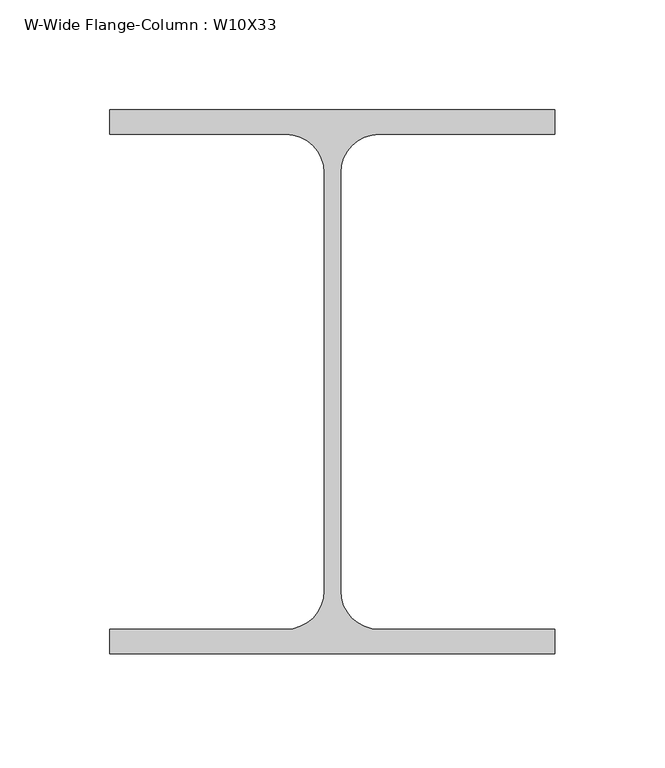
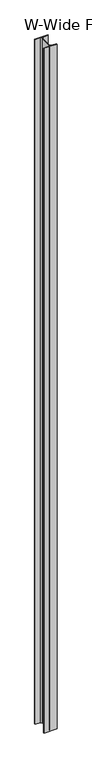
"""IFC4 building model written with IfcOpenShell, lengths in millimetres: column geometry, W-Wide Flange-Column : W10X33."""

from ifc_helpers import new_model, si_unit, point, frame, frame_2d, origin, place, context, project, spatial, polyline, circle_curve, trimmed, segment, composite_curve, outline, extrude, source, transform, mapped, element, save


def w_wide_flange_column_w10x33_06541e1f(model_context):
    return source(origin(), model_context, "Body", "SweptSolid", [
        extrude(outline(composite_curve([segment(polyline([(101.092, -123.571), (-101.092, -123.571), (-101.092, -112.522), (-21.209, -112.522)]), True, "CONTINUOUS"), segment(trimmed(circle_curve(frame_2d((-21.209, -94.996)), 17.526), [point((-21.209, -112.522))], [point((-3.683, -94.996))], True, "CARTESIAN"), True, "CONTINUOUS"), segment(polyline([(-3.683, -94.996), (-3.683, 94.996)]), True, "CONTINUOUS"), segment(trimmed(circle_curve(frame_2d((-21.209, 94.996)), 17.526), [point((-3.683, 94.996))], [point((-21.209, 112.522))], True, "CARTESIAN"), True, "CONTINUOUS"), segment(polyline([(-21.209, 112.522), (-101.092, 112.522), (-101.092, 123.571), (101.092, 123.571), (101.092, 112.522), (21.209, 112.522)]), True, "CONTINUOUS"), segment(trimmed(circle_curve(frame_2d((21.209, 94.996)), 17.526), [point((21.209, 112.522))], [point((3.683, 94.996))], True, "CARTESIAN"), True, "CONTINUOUS"), segment(polyline([(3.683, 94.996), (3.683, -94.996)]), True, "CONTINUOUS"), segment(trimmed(circle_curve(frame_2d((21.209, -94.996)), 17.526), [point((3.683, -94.996))], [point((21.209, -112.522))], True, "CARTESIAN"), True, "CONTINUOUS"), segment(polyline([(21.209, -112.522), (101.092, -112.522), (101.092, -123.571)]), True, "CONTINUOUS")], self_intersect=False)), frame((0.0, 0.0, 16408.4), z_axis=(0.0, 0.0, 1.0), x_axis=(1.0, 0.0, 0.0)), (0.0, 0.0, 1.0), 11176.0),
    ])


if __name__ == "__main__":
    model = new_model("IFC4")
    model_context = context("Model", 3, world=origin())
    ifc_project = project(units=[si_unit("LENGTHUNIT", "METRE", prefix="MILLI")], contexts=[model_context])
    site = spatial("IfcSite", under=ifc_project)
    building = spatial("IfcBuilding", under=site)
    placement = place(None, origin())
    w_wide_flange_column_w10x33_shape = w_wide_flange_column_w10x33_06541e1f(model_context)
    element("IfcColumn", 1, ObjectType="W-Wide Flange-Column : W10X33", at=placement, inside=building, context=model_context, shape_type="MappedRepresentation", body=[
        mapped(w_wide_flange_column_w10x33_shape, transform((0.0, 0.0, 0.0), x_axis=(1.0, 0.0, 0.0), y_axis=(0.0, 1.0, 0.0), z_axis=(0.0, 0.0, 1.0))),
    ])
    save(model, "model.ifc")

# Revit data of these elements
# Type "W-Wide Flange-Column : W10X33"
#   Assembly Code = "B10"
#   W = 33
#   bf = 0' - 7.96"
#   d = 0' - 9.73"
#   k = 0' - 1 1/8"
#   kr = 0' - 0.69"
#   tf = 0' - 0.435"
#   tw = 0' - 0.29"
#   A = 0.0674306 SF
#   Structural Material [instance default] = Steel ASTM A992
# Element 1 (IfcColumn, "W-Wide Flange-Column : W10X33")
#   Materials on its faces: "Steel ASTM A992"
# Materials
#   "Steel ASTM A992": class "Metal", colour RGB 199 199 199, transparency 0, Description = "Structural steel 50ksi", Cost = 0
